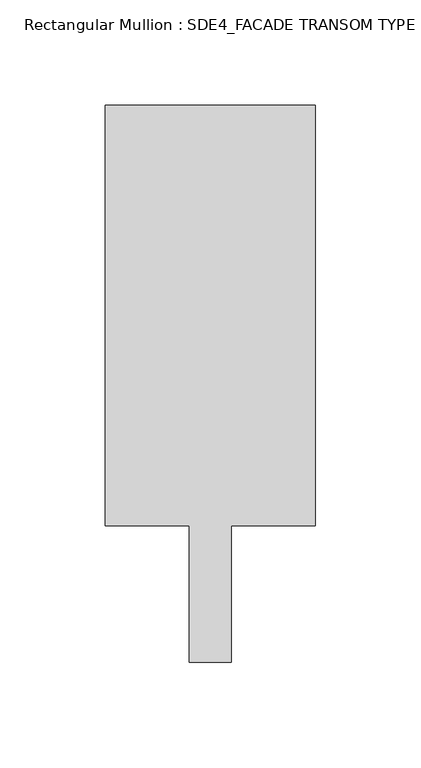
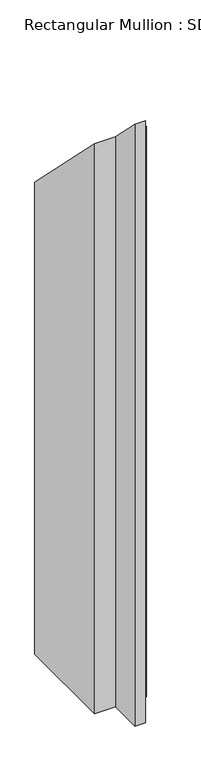
"""IFC4 building model written with IfcOpenShell, lengths in millimetres: member geometry, Rectangular Mullion : SDE4_FACADE TRANSOM TYPE 2."""

import ifcopenshell
import ifcopenshell.guid

model = None  # the IFC model being written
_history = None  # IfcOwnerHistory: only IFC2X3 demands one
_inside = {}  # id of a spatial element -> (the spatial element, [elements in it])
_under = {}  # id of a project, library or spatial element -> (it, [spatial elements below it])
_declared = {}  # id of a project -> (the project, [libraries it declares])
_typed = {}  # id of a type object -> (the type object, [elements of that type])
_made_of = {}  # id of a material, layer set ... -> (it, [elements and type objects made of it])


def new_model(schema):
    """Start an empty IFC model of exactly this schema.

    Asked for "IFC4X3", IfcOpenShell would pick the latest addendum, in which some entities
    have other attributes; the version numbers below select the first issue.
    IFC2X3 requires an IfcOwnerHistory on every rooted entity: one is made here for all.
    """
    global model, _history
    if schema == "IFC4X3":
        model = ifcopenshell.file(schema_version=(4, 3, 0, 0))
    else:
        model = ifcopenshell.file(schema=schema)
    _inside.clear()
    _under.clear()
    _declared.clear()
    _typed.clear()
    _made_of.clear()
    _history = None
    if model.schema == "IFC2X3":
        org = make("IfcOrganization", Name="unknown")
        user = make(
            "IfcPersonAndOrganization",
            ThePerson=make("IfcPerson", FamilyName="unknown"),
            TheOrganization=org,
        )
        app = make(
            "IfcApplication",
            ApplicationDeveloper=org,
            Version="unknown",
            ApplicationFullName="unknown",
            ApplicationIdentifier="unknown",
        )
        _history = make(
            "IfcOwnerHistory",
            OwningUser=user,
            OwningApplication=app,
            ChangeAction="ADDED",
            CreationDate=0,
        )
    return model


def make(cls, **values):
    """One entity of the class cls with the attributes given. An attribute that is None is left unset."""
    return model.create_entity(
        cls, **{name: value for name, value in values.items() if value is not None}
    )


def rooted(cls, **values):
    """An entity with a GlobalId (a new one), such as an element, a storey or a relation."""
    return make(cls, GlobalId=ifcopenshell.guid.new(), OwnerHistory=_history, **values)


def si_unit(unit_type, name, prefix=None):
    """IfcSIUnit, for example si_unit("LENGTHUNIT", "METRE", prefix="MILLI")."""
    return make("IfcSIUnit", UnitType=unit_type, Prefix=prefix, Name=name)


def assignment(units):
    """IfcUnitAssignment: the units of a project."""
    return None if units is None else make("IfcUnitAssignment", Units=units)


def point(xyz):
    """IfcCartesianPoint."""
    return None if xyz is None else make("IfcCartesianPoint", Coordinates=xyz)


def direction(xyz):
    """IfcDirection."""
    return None if xyz is None else make("IfcDirection", DirectionRatios=xyz)


def frame(location, z_axis=None, x_axis=None):
    """IfcAxis2Placement3D, a coordinate frame: its origin and axes. An axis left out is left unset."""
    return make(
        "IfcAxis2Placement3D",
        Location=point(location),
        Axis=direction(z_axis),
        RefDirection=direction(x_axis),
    )


def origin():
    """The frame at (0, 0, 0) with its axes left unset."""
    return frame((0.0, 0.0, 0.0))


def place(relative_to, where):
    """IfcLocalPlacement: puts the frame where relative to a parent placement (None: the world)."""
    return make(
        "IfcLocalPlacement", PlacementRelTo=relative_to, RelativePlacement=where
    )


def context(
    kind, dimensions, precision=None, world=None, true_north=None, identifier=None
):
    """IfcGeometricRepresentationContext, for example the 3D "Model" context."""
    return make(
        "IfcGeometricRepresentationContext",
        ContextIdentifier=identifier,
        ContextType=kind,
        CoordinateSpaceDimension=dimensions,
        Precision=precision,
        WorldCoordinateSystem=world,
        TrueNorth=true_north,
    )


def project(units=None, contexts=None):
    """IfcProject with its units and contexts."""
    return rooted(
        "IfcProject",
        Name="project",
        RepresentationContexts=contexts,
        UnitsInContext=assignment(units),
    )


def spatial(cls, under=None, at=None, **own):
    """A site, building, storey or space (cls), placed at a placement, below another one or the project."""
    s = rooted(cls, ObjectPlacement=at, **own)
    if under is not None:
        _under.setdefault(under.id(), (under, []))[1].append(s)
    return s


def faces_of(points, faces, orient=None, outer=None):
    """IfcFace entities. A face is a list of loops; a loop is a list of indices into points, from 0.

    orient and outer hold one flag for each loop. By default every Orientation is true, the
    first loop of a face is its IfcFaceOuterBound and the others are IfcFaceBound.
    """
    made = []
    for i, loops in enumerate(faces):
        bounds = []
        for j, loop in enumerate(loops):
            is_outer = j == 0 if outer is None else outer[i][j]
            bounds.append(
                make(
                    "IfcFaceOuterBound" if is_outer else "IfcFaceBound",
                    Bound=make("IfcPolyLoop", Polygon=[points[k] for k in loop]),
                    Orientation=True if orient is None else orient[i][j],
                )
            )
        made.append(make("IfcFace", Bounds=bounds))
    return made


def faceted_brep(points, faces, orient=None, outer=None, voids=None):
    """IfcFacetedBrep: a solid bounded by flat faces; with voids (closed shells), ...WithVoids."""
    shared = [point(p) for p in points]
    hull = make("IfcClosedShell", CfsFaces=faces_of(shared, faces, orient, outer))
    if voids is None:
        return make("IfcFacetedBrep", Outer=hull)
    return make(
        "IfcFacetedBrepWithVoids",
        Outer=hull,
        Voids=[
            make(cls, CfsFaces=faces_of(shared, fs, o, b)) for cls, fs, o, b in voids
        ],
    )


def shape(context_of_items, identifier, shape_type, items):
    """IfcShapeRepresentation: the items that make up one representation, for example the "Body"."""
    return make(
        "IfcShapeRepresentation",
        ContextOfItems=context_of_items,
        RepresentationIdentifier=identifier,
        RepresentationType=shape_type,
        Items=items,
    )


def source(mapping_origin, context_of_items, identifier, shape_type, items):
    """IfcRepresentationMap: a shape defined once, which mapped items show again and again."""
    return make(
        "IfcRepresentationMap",
        MappingOrigin=mapping_origin,
        MappedRepresentation=shape(context_of_items, identifier, shape_type, items),
    )


def transform(
    local_origin,
    x_axis=None,
    y_axis=None,
    z_axis=None,
    scale=None,
    scale2=None,
    scale3=None,
    uniform=True,
):
    """IfcCartesianTransformationOperator3D, or its non-uniform kind. x_axis, y_axis, z_axis: its Axis1, 2, 3."""
    if uniform:
        return make(
            "IfcCartesianTransformationOperator3D",
            Axis1=direction(x_axis),
            Axis2=direction(y_axis),
            LocalOrigin=point(local_origin),
            Scale=scale,
            Axis3=direction(z_axis),
        )
    return make(
        "IfcCartesianTransformationOperator3DnonUniform",
        Axis1=direction(x_axis),
        Axis2=direction(y_axis),
        LocalOrigin=point(local_origin),
        Scale=scale,
        Axis3=direction(z_axis),
        Scale2=scale2,
        Scale3=scale3,
    )


def mapped(mapping_source, mapping_target):
    """IfcMappedItem: shows the shape of a source again, moved by a transform."""
    return make(
        "IfcMappedItem", MappingSource=mapping_source, MappingTarget=mapping_target
    )


def made_of(thing, what):
    """Note that an element or type object is made of a material, layer set ...; save() writes the relation."""
    if what is not None:
        _made_of.setdefault(what.id(), (what, []))[1].append(thing)
    return thing


def element(
    cls,
    number,
    at=None,
    inside=None,
    cuts=None,
    type_object=None,
    material=None,
    context=None,
    identifier="Body",
    shape_type=None,
    held_by="IfcProductDefinitionShape",
    body=None,
    shapes=None,
    **own,
):
    """One element of the class cls, such as IfcWall. Its Tag is "e" and its number.

    at: its placement. inside: the storey or other place that contains it. cuts: it is an
    opening in that element (IfcRelVoidsElement). A single representation is given by context,
    identifier, shape_type and body (its items); several are given by shapes. held_by: the class
    of the entity that holds the representations. save() writes the other relations.
    """
    e = rooted(cls, Tag="e%d" % number, ObjectPlacement=at, **own)
    if body is not None:
        shapes = [shape(context, identifier, shape_type, body)]
    if shapes is not None:
        e.Representation = make(held_by, Representations=shapes)
    if inside is not None:
        _inside.setdefault(inside.id(), (inside, []))[1].append(e)
    if cuts is not None:
        rooted(
            "IfcRelVoidsElement", RelatingBuildingElement=cuts, RelatedOpeningElement=e
        )
    if type_object is not None:
        _typed.setdefault(type_object.id(), (type_object, []))[1].append(e)
    return made_of(e, material)


def aggregate(whole, parts):
    """IfcRelAggregates: a whole, such as a stair, and the parts it consists of."""
    return rooted("IfcRelAggregates", RelatingObject=whole, RelatedObjects=parts)


def save(model, path):
    """Write the relations noted so far, then the file.

    IfcRelAggregates (storeys below a building ...), IfcRelContainedInSpatialStructure (elements
    in a storey), IfcRelDefinesByType, IfcRelAssociatesMaterial and IfcRelDeclares: one each for
    every whole, place, type object, material and project.
    """
    for whole, parts in _under.values():
        aggregate(whole, parts)
    for where, things in _inside.values():
        rooted(
            "IfcRelContainedInSpatialStructure",
            RelatedElements=things,
            RelatingStructure=where,
        )
    for kind, things in _typed.values():
        rooted("IfcRelDefinesByType", RelatedObjects=things, RelatingType=kind)
    for what, things in _made_of.values():
        rooted("IfcRelAssociatesMaterial", RelatedObjects=things, RelatingMaterial=what)
    for by, libraries in _declared.values():
        rooted("IfcRelDeclares", RelatingContext=by, RelatedDefinitions=libraries)
    model.write(path)


def rectangular_mullion_sde4_facade_transom_type_2_a2326077(model_context):
    return source(origin(), model_context, "Body", "Brep", [
        faceted_brep([(50.0, 132.5, -1092.5), (50.0, -67.5, -1092.5), (10.0, -67.5, -1092.5), (10.0, -132.5, -1092.5), (-10.0, -132.5, -1092.5), (-10.0, -67.5, -1092.5), (-50.0, -67.5, -1092.5), (-50.0, 132.5, -1092.5), (-50.0, 132.5, -132.5), (50.0, 132.5, -132.5), (-50.0, -67.5, 67.5), (-10.0, -67.5, 67.5), (-10.0, -132.5, 132.5), (10.0, -132.5, 132.5), (10.0, -67.5, 67.5), (50.0, -67.5, 67.5)], [[[0, 1, 2, 3, 4, 5, 6, 7]], [[8, 9, 0, 7]], [[10, 8, 7, 6]], [[11, 10, 6, 5]], [[12, 11, 5, 4]], [[13, 12, 4, 3]], [[14, 13, 3, 2]], [[15, 14, 2, 1]], [[9, 15, 1, 0]], [[9, 8, 10, 11, 12, 13, 14, 15]]]),
    ])


if __name__ == "__main__":
    model = new_model("IFC4")
    model_context = context("Model", 3, world=origin())
    ifc_project = project(units=[si_unit("LENGTHUNIT", "METRE", prefix="MILLI")], contexts=[model_context])
    site = spatial("IfcSite", under=ifc_project)
    building = spatial("IfcBuilding", under=site)
    placement = place(None, origin())
    rectangular_mullion_sde4_facade_transom_type_2_shape = rectangular_mullion_sde4_facade_transom_type_2_a2326077(model_context)
    element("IfcMember", 1, ObjectType="Rectangular Mullion : SDE4_FACADE TRANSOM TYPE 2", at=placement, inside=building, context=model_context, shape_type="MappedRepresentation", body=[
        mapped(rectangular_mullion_sde4_facade_transom_type_2_shape, transform((0.0, 0.0, 0.0), x_axis=(1.0, 0.0, 0.0), y_axis=(0.0, 1.0, 0.0), z_axis=(0.0, 0.0, 1.0))),
    ])
    save(model, "model.ifc")

# Revit data of these elements
# Type "Rectangular Mullion : SDE4_FACADE TRANSOM TYPE 2"
#   built-in parameter 1007322 = 0.869423 (stored number, unit not read)
#   built-in parameter 1007321 = 0.164042 (stored number, unit not read)
#   built-in parameter 1007320 = 0.164042 (stored number, unit not read)
